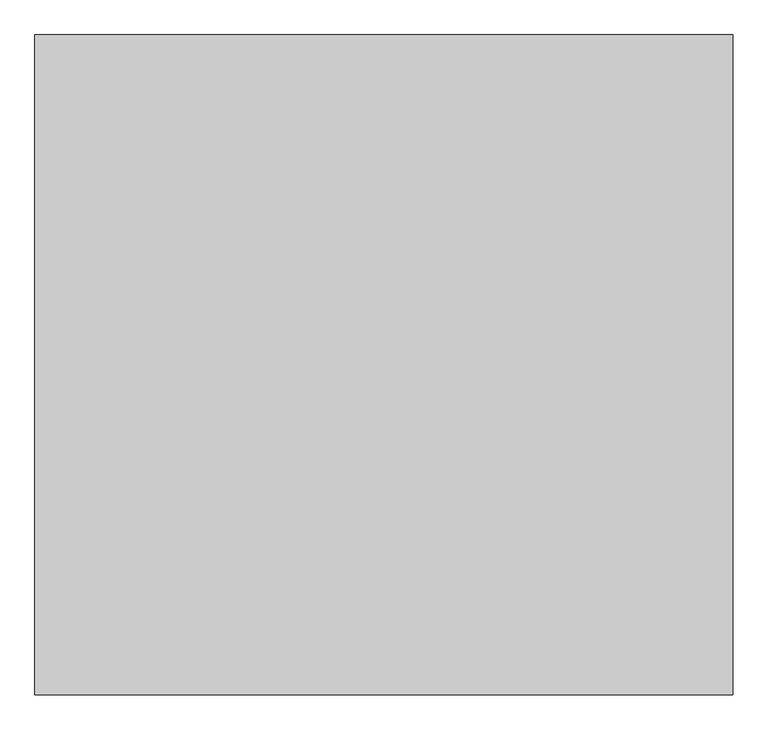
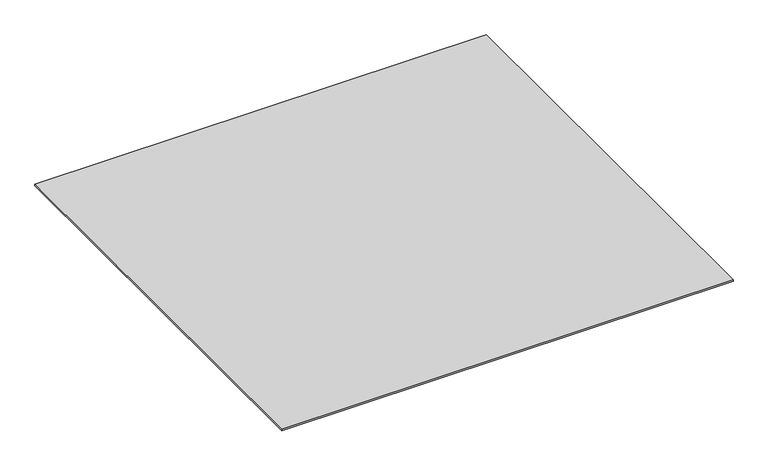
"""IFC4 building model written with IfcOpenShell, lengths in millimetres: proxy geometry, Generic Models 7:Generic Models 1:6:Generic Models 1:6 : Generic Models 7:Generic Models 1:337419:3 : Generic Models 7:Generic Models 1:6:Generic Models 1:6 : Generic Models 7:Generic Models 1:337419:312901."""

from ifc_helpers import new_model, si_unit, frame, origin, place, context, project, spatial, polyline, outline, extrude, source, transform, mapped, element, save


def generic_models_d607e0f8(model_context):
    return source(origin(), model_context, "Body", "SweptSolid", [
        extrude(outline(polyline([(602310.5867239, -536773.1913841), (602310.5867239, -578873.6913841), (557809.7867239, -578873.6913841), (557809.7867239, -536773.1913841), (602310.5867239, -536773.1913841)])), frame((0.0, 0.0, -158.1372439), z_axis=(0.0, 0.0, 1.0), x_axis=(1.0, 0.0, 0.0)), (0.0, 0.0, 1.0), 158.1372439),
    ])


if __name__ == "__main__":
    model = new_model("IFC4")
    model_context = context("Model", 3, world=origin())
    ifc_project = project(units=[si_unit("LENGTHUNIT", "METRE", prefix="MILLI")], contexts=[model_context])
    site = spatial("IfcSite", under=ifc_project)
    building = spatial("IfcBuilding", under=site)
    placement = place(None, origin())
    generic_models_shape = generic_models_d607e0f8(model_context)
    element("IfcBuildingElementProxy", 1, Name="Generic Models 7:Generic Models 1:6:Generic Models 1:6 : Generic Models 7:Generic Models 1:337419:3 : Generic Models 7:Generic Models 1:6:Generic Models 1:6 : Generic Models 7:Generic Models 1:337419:312901", ObjectType="Generic Models 7:Generic Models 1:6:Generic Models 1:6 : Generic Models 7:Generic Models 1:337419:3 : Generic Models 7:Generic Models 1:6:Generic Models 1:6 : Generic Models 7:Generic Models 1:337419:312901", at=placement, inside=building, context=model_context, shape_type="MappedRepresentation", body=[
        mapped(generic_models_shape, transform((0.0, 0.0, 0.0), x_axis=(1.0, 0.0, 0.0), y_axis=(0.0, 1.0, 0.0), z_axis=(0.0, 0.0, 1.0))),
    ])
    save(model, "model.ifc")

# Revit data of these elements
# Type "Generic Models 7:Generic Models 1:6:Generic Models 1:6 : Generic Models 7:Generic Models 1:337419:3 : Generic Models 7:Generic Models 1:6:Generic Models 1:6 : Generic Models 7:Generic Models 1:337419:312901"
#   NameOverride = "Generic Models 7:Generic Models 1:6:Generic Models 1:6 : Generic Models 7:Generic Models 1:337419:312901"
#   ObjectTypeOverride = "Generic Models 1:6 : Generic Models 7:Generic Models 1:337419"
#   Reference = "Generic Models 1"
#   Tag = "312901"
# Element 1 (IfcBuildingElementProxy, "Generic Models 7:Generic Models 1:6:Generic Models 1:6 : Generic Models 7:Generic Models 1:337419:3 : Generic Models 7:Generic Models 1:6:Generic Models 1:6 : Generic Models 7:Generic Models 1:337419:312901")
#   Materials on its faces: "CONCRETE SLAB - SEE STRUCT DWGS."
# Materials
#   "CONCRETE SLAB - SEE STRUCT DWGS.": class "Concrete", colour RGB 115 116 108, transparency 0, Description = "Lightweight concrete", Cost = 0
